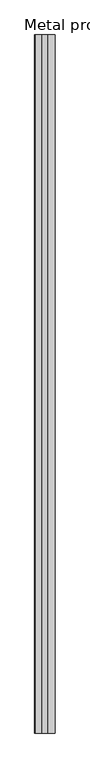
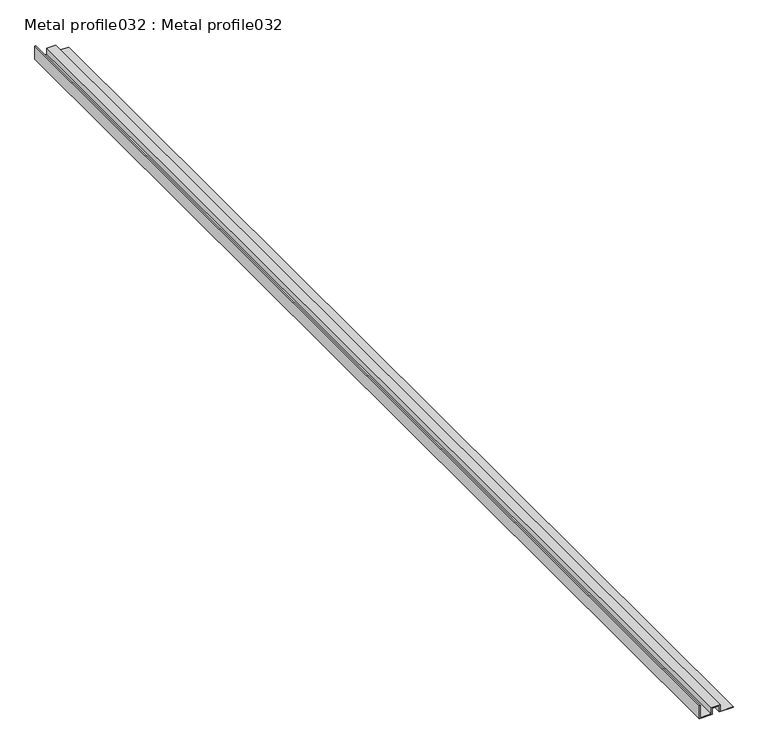
"""IFC4 building model written with IfcOpenShell, lengths in millimetres: proxy geometry, Metal profile032 : Metal profile032."""

from ifc_helpers import new_model, si_unit, frame, origin, place, context, project, spatial, polyline, outline, extrude, source, transform, mapped, element, save


def metal_profile032_metal_profile032_b7ba3d6c(model_context):
    return source(origin(), model_context, "Body", "SweptSolid", [
        extrude(outline(polyline([(39543.8875708, -9915.4255764), (39543.8875708, -9893.2005764), (39555.3175708, -9893.2005764), (39555.3175708, -9880.5005764), (39543.8875708, -9880.5005764), (39543.8875708, -9856.7873925), (39545.1675708, -9856.7873925), (39545.1675708, -9879.2205764), (39556.5975708, -9879.2205764), (39556.5975708, -9894.4805764), (39545.1675708, -9894.4805764), (39545.1675708, -9914.1455764), (39567.6883323, -9914.1455764), (39567.6883323, -9915.4255764), (39543.8875708, -9915.4255764)])), frame((0.0, 7982.1531721, 0.0), z_axis=(0.0, 1.0, 0.0), x_axis=(0.0, 0.0, 1.0)), (0.0, 0.0, 1.0), 2000.0),
    ])


if __name__ == "__main__":
    model = new_model("IFC4")
    model_context = context("Model", 3, world=origin())
    ifc_project = project(units=[si_unit("LENGTHUNIT", "METRE", prefix="MILLI")], contexts=[model_context])
    site = spatial("IfcSite", under=ifc_project)
    building = spatial("IfcBuilding", under=site)
    placement = place(None, origin())
    metal_profile032_metal_profile032_shape = metal_profile032_metal_profile032_b7ba3d6c(model_context)
    element("IfcBuildingElementProxy", 1, Name="Metal profile032 : Metal profile032", ObjectType="Metal profile032 : Metal profile032", at=placement, inside=building, context=model_context, shape_type="MappedRepresentation", body=[
        mapped(metal_profile032_metal_profile032_shape, transform((0.0, 0.0, 0.0), x_axis=(1.0, 0.0, 0.0), y_axis=(0.0, 1.0, 0.0), z_axis=(0.0, 0.0, 1.0))),
    ])
    save(model, "model.ifc")

# Revit data of these elements
# Type "Metal profile032 : Metal profile032"
#   NameOverride = "Metal profile032"
# Element 1 (IfcBuildingElementProxy, "Metal profile032 : Metal profile032")
#   Materials on its faces: "16 GA. COPPER SOFFIT DRIP SCREED"
# Materials
#   "16 GA. COPPER SOFFIT DRIP SCREED": class "Unassigned", colour RGB 255 217 0, transparency 0
